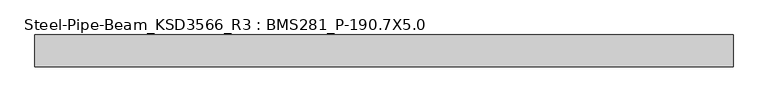
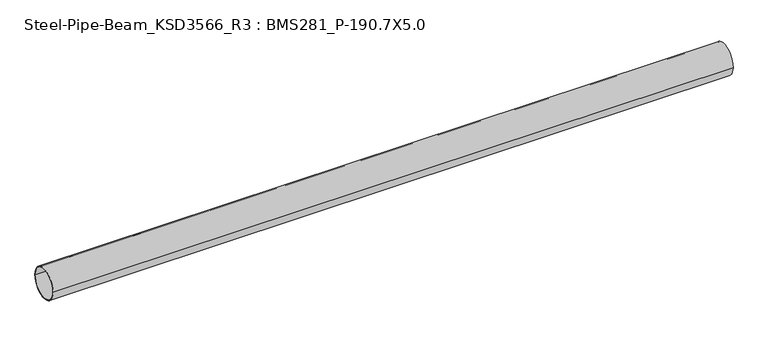
"""IFC4 building model written with IfcOpenShell, lengths in millimetres: member geometry, Steel-Pipe-Beam_KSD3566_R3 : BMS281_P-190.7X5.0."""

from ifc_helpers import new_model, si_unit, point, frame, origin, origin_2d, place, context, project, spatial, circle_curve, trimmed, segment, composite_curve, outline, extrude, source, transform, mapped, element, save


def steel_pipe_beam_ksd3566_r3_bms281_p_190_7x5_0_63678a68(model_context):
    return source(origin(), model_context, "Body", "SweptSolid", [
        extrude(outline(composite_curve([segment(trimmed(circle_curve(origin_2d(), 95.35), [point((-95.35, 0.0))], [point((95.35, 0.0))], False, "CARTESIAN"), True, "CONTINUOUS"), segment(trimmed(circle_curve(origin_2d(), 95.35), [point((95.35, 0.0))], [point((-95.35, 0.0))], False, "CARTESIAN"), True, "CONTINUOUS")], self_intersect=False), holes=[composite_curve([segment(trimmed(circle_curve(origin_2d(), 90.35), [point((90.35, 0.0))], [point((-90.35, 0.0))], True, "CARTESIAN"), True, "CONTINUOUS"), segment(trimmed(circle_curve(origin_2d(), 90.35), [point((-90.35, 0.0))], [point((90.35, 0.0))], True, "CARTESIAN"), True, "CONTINUOUS")], self_intersect=False)]), frame((-2106.2716567, 0.0, 0.0), z_axis=(1.0, 0.0, 0.0), x_axis=(0.0, 1.0, 0.0)), (0.0, 0.0, 1.0), 4152.4090653),
    ])


if __name__ == "__main__":
    model = new_model("IFC4")
    model_context = context("Model", 3, world=origin())
    ifc_project = project(units=[si_unit("LENGTHUNIT", "METRE", prefix="MILLI")], contexts=[model_context])
    site = spatial("IfcSite", under=ifc_project)
    building = spatial("IfcBuilding", under=site)
    placement = place(None, origin())
    steel_pipe_beam_ksd3566_r3_bms281_p_190_7x5_0_shape = steel_pipe_beam_ksd3566_r3_bms281_p_190_7x5_0_63678a68(model_context)
    element("IfcMember", 1, ObjectType="Steel-Pipe-Beam_KSD3566_R3 : BMS281_P-190.7X5.0", at=placement, inside=building, context=model_context, shape_type="MappedRepresentation", body=[
        mapped(steel_pipe_beam_ksd3566_r3_bms281_p_190_7x5_0_shape, transform((0.0, 0.0, 0.0), x_axis=(1.0, 0.0, 0.0), y_axis=(0.0, 1.0, 0.0), z_axis=(0.0, 0.0, 1.0))),
    ])
    save(model, "model.ifc")

# Revit data of these elements
# Type "Steel-Pipe-Beam_KSD3566_R3 : BMS281_P-190.7X5.0"
#   Keynote = "P-190.7X5.0"
#   SteelWeight = "Light"
#   t = 0.0050 m
#   Surface Area = 0.599102 m²/m
#   Section Area = 29.1697 cm²
#   Mass per Unit Length = 22.8982 kg/m
#   Length [instance default] = 1.5000 m
#   D = 0.1907 m
#   hec_material4 [instance default] = none
#   hec_material3 [instance default] = none
#   hec_material2 [instance default] = none
#   hec_material1 [instance default] = none
#   Structural Material [instance default] = Steel, 45-345
#   Assembly Code = ""
# Element 1 (IfcMember, "Steel-Pipe-Beam_KSD3566_R3 : BMS281_P-190.7X5.0")
#   Structural Material = none
# Materials
#   "Steel, 45-345": class "Metal", colour RGB 189 187 185, transparency 0, Description = "Steel 345 MPa", Cost = 0
